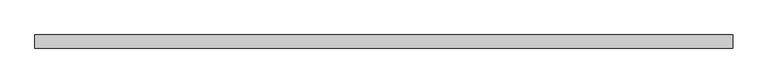
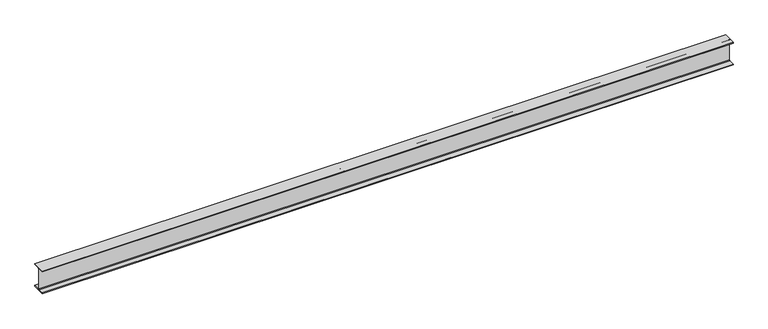
"""IFC4 building model written with IfcOpenShell, lengths in millimetres: beam geometry, Old_Steel Beam_H-KSD3502 : H_SB_ASB_H-300×300x10x15."""

from ifc_helpers import new_model, si_unit, point, frame, frame_2d, origin, place, context, project, spatial, polyline, circle_curve, trimmed, segment, composite_curve, outline, extrude, source, transform, mapped, element, save


def beam_97b2203e(model_context):
    return source(origin(), model_context, "Body", "SweptSolid", [
        extrude(outline(composite_curve([segment(polyline([(82.5, -141.5), (82.5, -151.7), (-82.5, -151.7), (-82.5, -141.5), (-11.9, -141.5)]), True, "CONTINUOUS"), segment(trimmed(circle_curve(frame_2d((-11.9, -132.6)), 8.9), [point((-11.9, -141.5))], [point((-3.0, -132.6))], True, "CARTESIAN"), True, "CONTINUOUS"), segment(polyline([(-3.0, -132.6), (-3.0, 132.6)]), True, "CONTINUOUS"), segment(trimmed(circle_curve(frame_2d((-11.9, 132.6)), 8.9), [point((-3.0, 132.6))], [point((-11.9, 141.5))], True, "CARTESIAN"), True, "CONTINUOUS"), segment(polyline([(-11.9, 141.5), (-82.5, 141.5), (-82.5, 151.7), (82.5, 151.7), (82.5, 141.5), (11.9, 141.5)]), True, "CONTINUOUS"), segment(trimmed(circle_curve(frame_2d((11.9, 132.6)), 8.9), [point((11.9, 141.5))], [point((3.0, 132.6))], True, "CARTESIAN"), True, "CONTINUOUS"), segment(polyline([(3.0, 132.6), (3.0, -132.6)]), True, "CONTINUOUS"), segment(trimmed(circle_curve(frame_2d((11.9, -132.6)), 8.9), [point((3.0, -132.6))], [point((11.9, -141.5))], True, "CARTESIAN"), True, "CONTINUOUS"), segment(polyline([(11.9, -141.5), (82.5, -141.5)]), True, "CONTINUOUS")], self_intersect=False)), frame((-4272.9251782, 0.0, 0.0), z_axis=(1.0, 0.0, 0.0), x_axis=(0.0, 1.0, 0.0)), (0.0, 0.0, 1.0), 8795.3692077),
    ])


if __name__ == "__main__":
    model = new_model("IFC4")
    model_context = context("Model", 3, world=origin())
    ifc_project = project(units=[si_unit("LENGTHUNIT", "METRE", prefix="MILLI")], contexts=[model_context])
    site = spatial("IfcSite", under=ifc_project)
    building = spatial("IfcBuilding", under=site)
    placement = place(None, origin())
    beam_shape = beam_97b2203e(model_context)
    element("IfcBeam", 1, ObjectType="Old_Steel Beam_H-KSD3502 : H_SB_ASB_H-300×300x10x15", at=placement, inside=building, context=model_context, shape_type="MappedRepresentation", body=[
        mapped(beam_shape, transform((0.0, 0.0, 0.0), x_axis=(1.0, 0.0, 0.0), y_axis=(0.0, 1.0, 0.0), z_axis=(0.0, 0.0, 1.0))),
    ])
    save(model, "model.ifc")

# Revit data of these elements
# Type "Old_Steel Beam_H-KSD3502 : H_SB_ASB_H-300×300x10x15"
#   Width = 30.0 cm
#   Web Thickness = 1.0 cm
#   Web Fillet = 1.8 cm
#   Warping Constant = 1370670.0 cm⁶
#   Torsional Moment of Inertia = 77.00 cm⁴
#   Torsional Modulus = 1.0 cm³
#   Section Area = 119.8 cm²
#   Plastic Modulus weak axis = 684.0 cm³
#   Plastic Modulus strong axis = 1500.0 cm³
#   Perimeter = 1.75 m²/m
#   Nominal Weight = 94.00 kgf/m
#   Moment of Inertia weak axis = 6750.00 cm⁴
#   Moment of Inertia strong axis = 20400.00 cm⁴
#   Height = 30.0 cm
#   Flange Thickness = 1.5 cm
#   Elastic Modulus weak axis = 450.0 cm³
#   Elastic Modulus strong axis = 1360.0 cm³
#   Centroid Vertical = 15.0 cm
#   Centroid Horizontal = 15.0 cm
#   Length [instance default] = 1.5240 m
#   Structural Material [instance default] = Steel, 45-345
#   Assembly Code = ""
# Element 1 (IfcBeam, "Old_Steel Beam_H-KSD3502 : H_SB_ASB_H-300×300x10x15")
#   Structural Material = none
# Materials
#   "Steel, 45-345": class "Metal", colour RGB 189 187 185, transparency 0, Description = "Steel 345 MPa", Cost = 0
